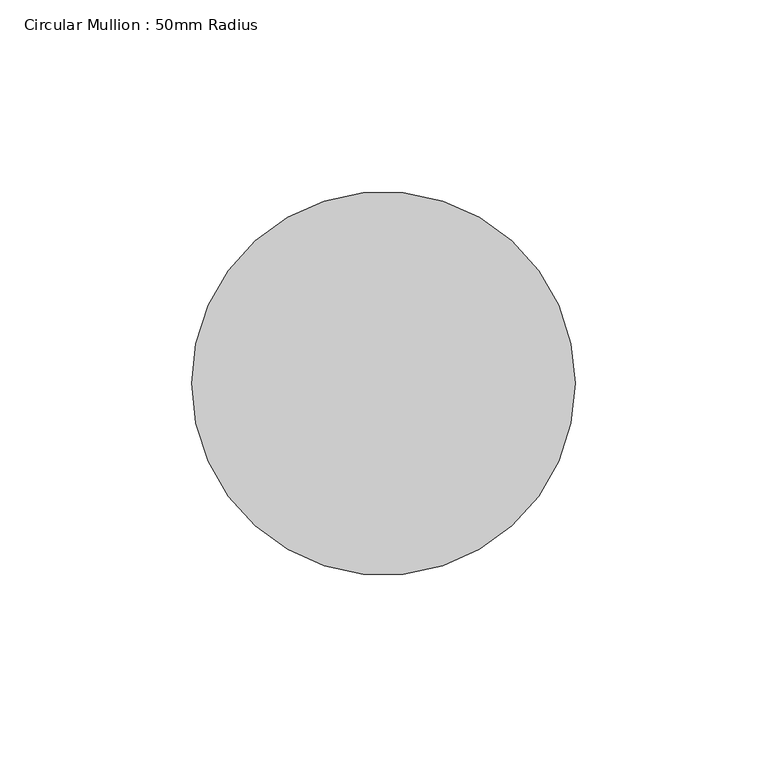
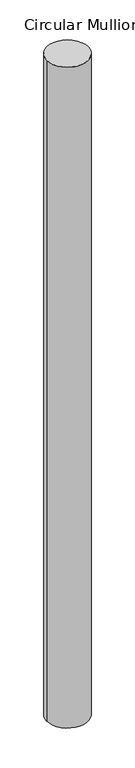
"""IFC4 building model written with IfcOpenShell, lengths in millimetres: member geometry, Circular Mullion : 50mm Radius."""

from ifc_helpers import new_model, si_unit, point, frame, origin, origin_2d, place, context, project, spatial, circle_curve, trimmed, segment, composite_curve, outline, extrude, source, transform, mapped, element, save


def circular_mullion_50mm_radius_89d2e96e(model_context):
    return source(origin(), model_context, "Body", "SweptSolid", [
        extrude(outline(composite_curve([segment(trimmed(circle_curve(origin_2d(), 50.0), [point((50.0, 0.0))], [point((-50.0, 0.0))], False, "CARTESIAN"), True, "CONTINUOUS"), segment(trimmed(circle_curve(origin_2d(), 50.0), [point((-50.0, 0.0))], [point((50.0, 0.0))], False, "CARTESIAN"), True, "CONTINUOUS")], self_intersect=False)), frame((0.0, 0.0, -1693.1656506), z_axis=(0.0, 0.0, 1.0), x_axis=(1.0, 0.0, 0.0)), (0.0, 0.0, 1.0), 1693.1656506),
    ])


if __name__ == "__main__":
    model = new_model("IFC4")
    model_context = context("Model", 3, world=origin())
    ifc_project = project(units=[si_unit("LENGTHUNIT", "METRE", prefix="MILLI")], contexts=[model_context])
    site = spatial("IfcSite", under=ifc_project)
    building = spatial("IfcBuilding", under=site)
    placement = place(None, origin())
    circular_mullion_50mm_radius_shape = circular_mullion_50mm_radius_89d2e96e(model_context)
    element("IfcMember", 1, ObjectType="Circular Mullion : 50mm Radius", at=placement, inside=building, context=model_context, shape_type="MappedRepresentation", body=[
        mapped(circular_mullion_50mm_radius_shape, transform((0.0, 0.0, 0.0), x_axis=(1.0, 0.0, 0.0), y_axis=(0.0, 1.0, 0.0), z_axis=(0.0, 0.0, 1.0))),
    ])
    save(model, "model.ifc")

# Revit data of these elements
# Type "Circular Mullion : 50mm Radius"
#   built-in parameter 1007350 = 0.164042 (stored number, unit not read)
# Element 1 (IfcMember, "Circular Mullion : 50mm Radius")
#   Materials on its faces: "Aluminium"
# Materials
#   "Aluminium": class "Metal", colour RGB 247 247 247, transparency 0, Description = "Aluminium 6061", Cost = 0
